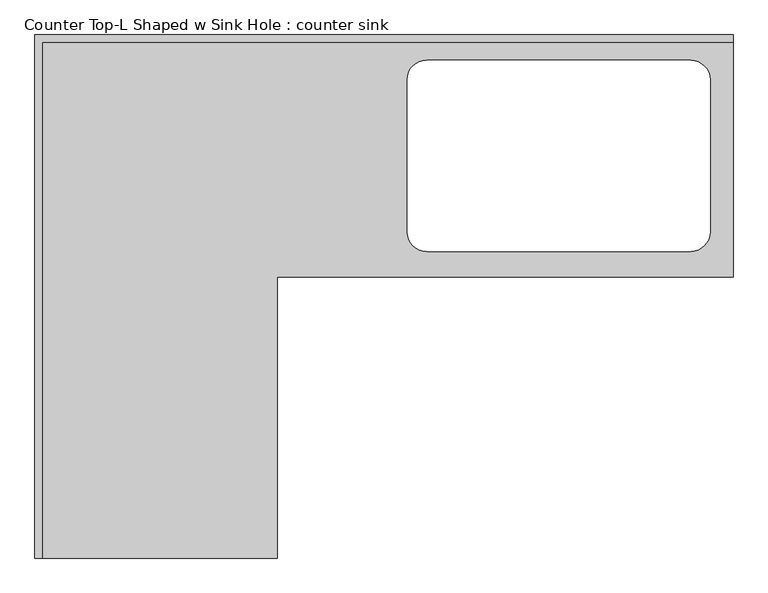
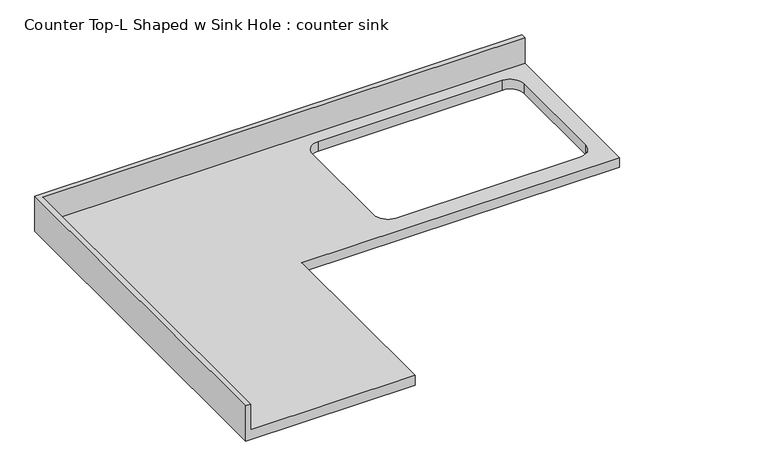
"""IFC4 building model written with IfcOpenShell, lengths in millimetres: furniture geometry, Counter Top-L Shaped w Sink Hole : counter sink."""

from ifc_helpers import new_model, si_unit, frame, origin, place, context, project, spatial, polyline, circle_curve, source, transform, mapped, element, save
from ifc_brep_helpers import plane_surface, revolved_surface, advanced_brep


def counter_top_l_shaped_w_sink_hole_counter_sink_67ca0d19(model_context):
    return source(origin(), model_context, "Body", "AdvancedBrep", [
        advanced_brep(
        [(-565.4622951, -1371.6, 914.4), (-565.4622951, -635.0, 914.4), (628.3377049, -635.0, 914.4), (628.3377049, -19.05, 914.4), (-1181.4122951, -19.05, 914.4), (-1181.4122951, -1371.6, 914.4), (517.2599348, -66.5566014, 914.4), (568.0599348, -117.3566014, 914.4), (568.0599348, -516.756388, 914.4), (517.2599348, -567.556388, 914.4), (-174.6245416, -567.556388, 914.4), (-225.4245416, -516.756388, 914.4), (-225.4245416, -117.3566014, 914.4), (-174.6245416, -66.5566014, 914.4), (628.3377049, 0.0, 876.3), (628.3377049, -635.0, 876.3), (-565.4622951, -635.0, 876.3), (-565.4622951, -1371.6, 876.3), (-1200.4622951, -1371.6, 876.3), (-1200.4622951, 0.0, 876.3), (517.2599348, -66.5566014, 876.3), (-174.6245416, -66.5566014, 876.3), (-225.4245416, -117.3566014, 876.3), (-225.4245416, -516.756388, 876.3), (-174.6245416, -567.556388, 876.3), (517.2599348, -567.556388, 876.3), (568.0599348, -516.756388, 876.3), (568.0599348, -117.3566014, 876.3), (-1200.4622951, 0.0, 1016.0), (628.3377049, 0.0, 1016.0), (-1200.4622951, -1371.6, 1016.0), (-1181.4122951, -1371.6, 1016.0), (628.3377049, -19.05, 1016.0), (-1181.4122951, -19.05, 1016.0)],
        [
            (0, 1),
            (1, 2),
            (2, 3),
            (3, 4),
            (4, 5),
            (5, 0),
            (6, 7, circle_curve(frame((517.2599348, -117.3566014, 914.4), z_axis=(0.0, 0.0, -1.0), x_axis=(1.0, 0.0, 0.0)), 50.8)),
            (7, 8),
            (8, 9, circle_curve(frame((517.2599348, -516.756388, 914.4), z_axis=(0.0, 0.0, -1.0), x_axis=(1.0, 0.0, 0.0)), 50.8)),
            (9, 10),
            (10, 11, circle_curve(frame((-174.6245416, -516.756388, 914.4), z_axis=(0.0, 0.0, -1.0), x_axis=(1.0, 0.0, 0.0)), 50.8)),
            (11, 12),
            (12, 13, circle_curve(frame((-174.6245416, -117.3566014, 914.4), z_axis=(0.0, 0.0, -1.0), x_axis=(1.0, 0.0, 0.0)), 50.8)),
            (13, 6),
            (14, 15),
            (15, 16),
            (16, 17),
            (17, 18),
            (18, 19),
            (19, 14),
            (20, 21),
            (21, 22, circle_curve(frame((-174.6245416, -117.3566014, 876.3), z_axis=(0.0, 0.0, 1.0), x_axis=(1.0, 0.0, 0.0)), 50.8)),
            (22, 23),
            (23, 24, circle_curve(frame((-174.6245416, -516.756388, 876.3), z_axis=(0.0, 0.0, 1.0), x_axis=(1.0, 0.0, 0.0)), 50.8)),
            (24, 25),
            (25, 26, circle_curve(frame((517.2599348, -516.756388, 876.3), z_axis=(0.0, 0.0, 1.0), x_axis=(1.0, 0.0, 0.0)), 50.8)),
            (26, 27),
            (27, 20, circle_curve(frame((517.2599348, -117.3566014, 876.3), z_axis=(0.0, 0.0, 1.0), x_axis=(1.0, 0.0, 0.0)), 50.8)),
            (19, 28),
            (28, 29),
            (29, 14),
            (18, 30),
            (30, 28),
            (17, 0),
            (5, 31),
            (31, 30),
            (16, 1),
            (15, 2),
            (29, 32),
            (32, 3),
            (6, 20),
            (27, 7),
            (26, 8),
            (25, 9),
            (24, 10),
            (23, 11),
            (22, 12),
            (21, 13),
            (31, 33),
            (33, 32),
            (33, 4),
        ],
        [
            plane_surface(frame((-1200.4622951, 0.0, 914.4), z_axis=(0.0, 0.0, 1.0), x_axis=(-1.0, 0.0, 0.0))),
            plane_surface(frame((-1200.4622951, 0.0, 876.3), z_axis=(0.0, 0.0, -1.0), x_axis=(1.0, 0.0, 0.0))),
            plane_surface(frame((628.3377049, 0.0, 914.4), z_axis=(0.0, 1.0, 0.0), x_axis=(0.0, 0.0, -1.0))),
            plane_surface(frame((-1200.4622951, 0.0, 914.4), z_axis=(-1.0, 0.0, 0.0), x_axis=(0.0, 0.0, -1.0))),
            plane_surface(frame((-1200.4622951, -1371.6, 914.4), z_axis=(0.0, -1.0, 0.0), x_axis=(0.0, 0.0, -1.0))),
            plane_surface(frame((-565.4622951, -1371.6, 914.4), z_axis=(1.0, 0.0, 0.0), x_axis=(0.0, 0.0, -1.0))),
            plane_surface(frame((-565.4622951, -635.0, 914.4), z_axis=(0.0, -1.0, 0.0), x_axis=(0.0, 0.0, -1.0))),
            plane_surface(frame((628.3377049, -635.0, 914.4), z_axis=(1.0, 0.0, 0.0), x_axis=(0.0, 0.0, -1.0))),
            revolved_surface(polyline([(568.0599348, -117.3566014, 876.3), (568.0599348, -117.3566014, 914.4)]), (517.2599348, -117.3566014, 0.0), (0.0, 0.0, -1.0)),
            plane_surface(frame((568.0599348, -117.3566014, 914.4), z_axis=(-1.0, 0.0, 0.0), x_axis=(0.0, 0.0, -1.0))),
            revolved_surface(polyline([(568.0599348, -516.756388, 876.3), (568.0599348, -516.756388, 914.4)]), (517.2599348, -516.756388, 0.0), (0.0, 0.0, -1.0)),
            plane_surface(frame((517.2599348, -567.556388, 914.4), z_axis=(0.0, 1.0, 0.0), x_axis=(0.0, 0.0, -1.0))),
            revolved_surface(polyline([(-123.82454159999999, -516.756388, 876.3), (-123.82454159999999, -516.756388, 914.4)]), (-174.6245416, -516.756388, 0.0), (0.0, 0.0, -1.0)),
            plane_surface(frame((-225.4245416, -516.756388, 914.4), z_axis=(1.0, 0.0, 0.0), x_axis=(0.0, 0.0, -1.0))),
            revolved_surface(polyline([(-123.82454159999999, -117.3566014, 876.3), (-123.82454159999999, -117.3566014, 914.4)]), (-174.6245416, -117.3566014, 0.0), (0.0, 0.0, -1.0)),
            plane_surface(frame((-174.6245416, -66.5566014, 914.4), z_axis=(0.0, -1.0, 0.0), x_axis=(0.0, 0.0, -1.0))),
            plane_surface(frame((-1200.4622951, 0.0, 1016.0), z_axis=(0.0, 0.0, 1.0), x_axis=(0.0, -1.0, 0.0))),
            plane_surface(frame((-1200.4622951, -19.05, 1016.0), z_axis=(0.0, -1.0, 0.0), x_axis=(0.0, 0.0, -1.0))),
            plane_surface(frame((-1181.4122951, -1371.6, 1016.0), z_axis=(1.0, 0.0, 0.0), x_axis=(0.0, 0.0, -1.0))),
        ],
        [
            (0, [[1, 2, 3, 4, 5, 6], [7, 8, 9, 10, 11, 12, 13, 14]]),
            (1, [[15, 16, 17, 18, 19, 20], [21, 22, 23, 24, 25, 26, 27, 28]]),
            (2, [[-20, 29, 30, 31]]),
            (3, [[-19, 32, 33, -29]]),
            (4, [[-32, -18, 34, -6, 35, 36]]),
            (5, [[-1, -34, -17, 37]]),
            (6, [[-2, -37, -16, 38]]),
            (7, [[-15, -31, 39, 40, -3, -38]]),
            (8, [[-7, 41, -28, 42]]),
            (9, [[-8, -42, -27, 43]]),
            (10, [[-9, -43, -26, 44]]),
            (11, [[-10, -44, -25, 45]]),
            (12, [[-11, -45, -24, 46]]),
            (13, [[-12, -46, -23, 47]]),
            (14, [[-13, -47, -22, 48]]),
            (15, [[-14, -48, -21, -41]]),
            (16, [[-33, -36, 49, 50, -39, -30]]),
            (17, [[-40, -50, 51, -4]]),
            (18, [[-49, -35, -5, -51]]),
        ],
    ),
    ])


if __name__ == "__main__":
    model = new_model("IFC4")
    model_context = context("Model", 3, world=origin())
    ifc_project = project(units=[si_unit("LENGTHUNIT", "METRE", prefix="MILLI")], contexts=[model_context])
    site = spatial("IfcSite", under=ifc_project)
    building = spatial("IfcBuilding", under=site)
    placement = place(None, origin())
    counter_top_l_shaped_w_sink_hole_counter_sink_shape = counter_top_l_shaped_w_sink_hole_counter_sink_67ca0d19(model_context)
    element("IfcFurniture", 1, ObjectType="Counter Top-L Shaped w Sink Hole : counter sink", at=placement, inside=building, context=model_context, shape_type="MappedRepresentation", body=[
        mapped(counter_top_l_shaped_w_sink_hole_counter_sink_shape, transform((0.0, 0.0, 0.0), x_axis=(1.0, 0.0, 0.0), y_axis=(0.0, 1.0, 0.0), z_axis=(0.0, 0.0, 1.0))),
    ])
    save(model, "model.ifc")

# Revit data of these elements
# Type "Counter Top-L Shaped w Sink Hole : counter sink"
#   Assembly Code = "C1030400"
#   Counter Thickness = 0' - 1 1/2"
#   Depth = 2' - 1"
#   Height = 3' - 0"
#   Length - Leg 1 [instance default] = 8' - 0"
#   Length - Leg 2 [instance default] = 6' - 0"
#   Sink Location [instance default] = 2' - 10 1/2"
#   Sink Location To Wall [instance default] = 0' - 6"
#   Sink Opening Depth [instance default] = 1' - 3"
#   Sink Opening Width [instance default] = 2' - 3"
#   Counter Top Material = Counter Top
#   Default Elevation = 0
# Element 1 (IfcFurniture, "Counter Top-L Shaped w Sink Hole : counter sink")
#   Length - Leg 1 = 6' - 0"
#   Length - Leg 2 = 4' - 6"
#   Sink Location = 3' - 2.38731"
#   Sink Location To Wall = 0' - 2.62034"
#   Sink Opening Depth = 1' - 7.7244"
#   Sink Opening Width = 2' - 7.23955"
#   Materials on its faces: "Counter Top"
# Materials
#   "Counter Top": class "Wood", colour RGB 226 177 128, transparency 0
